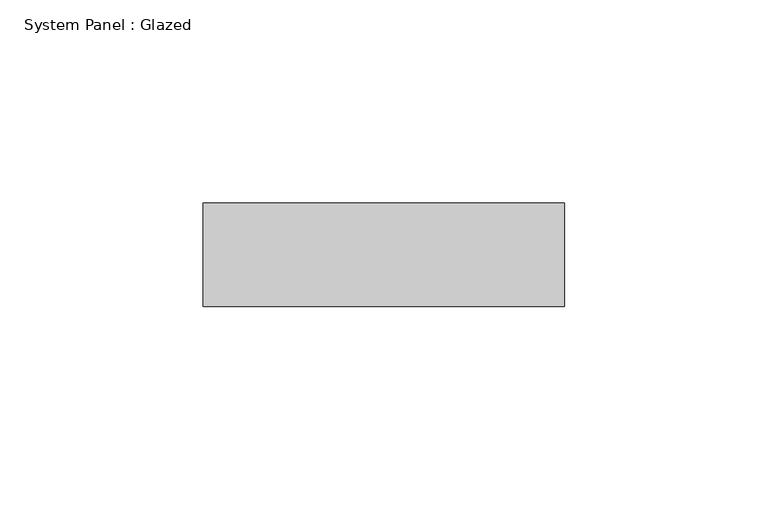
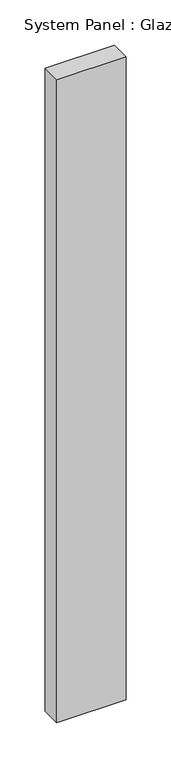
"""IFC4 building model written with IfcOpenShell, lengths in millimetres: plate geometry, System Panel : Glazed."""

from ifc_helpers import new_model, si_unit, origin, origin_with_axes, place, context, project, spatial, polyline, outline, extrude, source, transform, mapped, element, save


def system_panel_glazed_47952c94(model_context):
    return source(origin(), model_context, "Body", "SweptSolid", [
        extrude(outline(polyline([(44.45, 19.05), (-44.45, 19.05), (-44.45, 44.45), (44.45, 44.45), (44.45, 19.05)])), origin_with_axes(), (0.0, 0.0, 1.0), 869.95),
    ])


if __name__ == "__main__":
    model = new_model("IFC4")
    model_context = context("Model", 3, world=origin())
    ifc_project = project(units=[si_unit("LENGTHUNIT", "METRE", prefix="MILLI")], contexts=[model_context])
    site = spatial("IfcSite", under=ifc_project)
    building = spatial("IfcBuilding", under=site)
    placement = place(None, origin())
    system_panel_glazed_shape = system_panel_glazed_47952c94(model_context)
    element("IfcPlate", 1, ObjectType="System Panel : Glazed", at=placement, inside=building, context=model_context, shape_type="MappedRepresentation", body=[
        mapped(system_panel_glazed_shape, transform((0.0, 0.0, 0.0), x_axis=(1.0, 0.0, 0.0), y_axis=(0.0, 1.0, 0.0), z_axis=(0.0, 0.0, 1.0))),
    ])
    save(model, "model.ifc")

# Revit data of these elements
# Element 1 (IfcPlate, "System Panel : Glazed")
#   Materials on its faces: "Glass"
# Materials
#   "Glass": class "Glass", colour RGB 0 128 192, transparency 0.75
